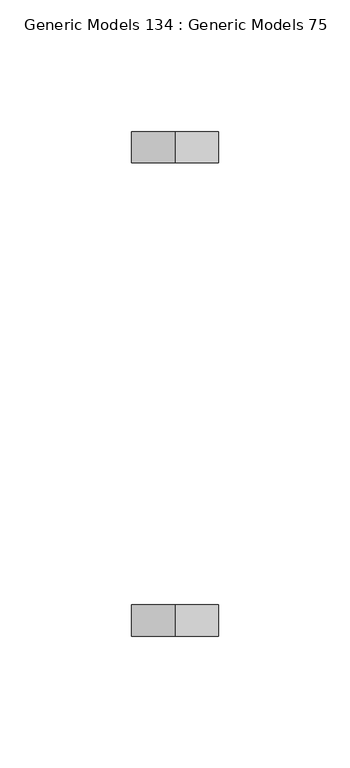
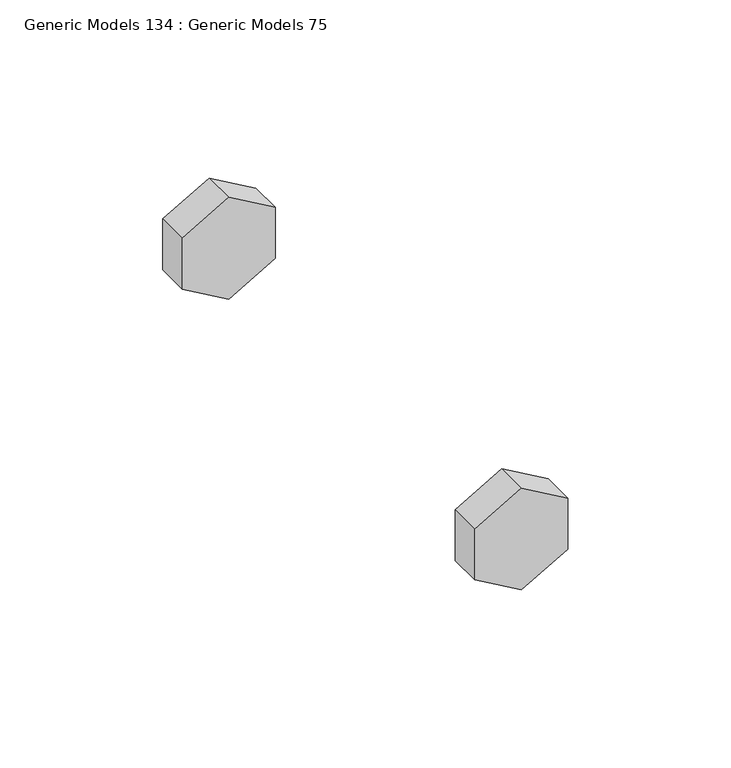
"""IFC4 building model written with IfcOpenShell, lengths in millimetres: proxy geometry, Generic Models 134 : Generic Models 75."""

import ifcopenshell
import ifcopenshell.guid

model = None  # the IFC model being written
_history = None  # IfcOwnerHistory: only IFC2X3 demands one
_inside = {}  # id of a spatial element -> (the spatial element, [elements in it])
_under = {}  # id of a project, library or spatial element -> (it, [spatial elements below it])
_declared = {}  # id of a project -> (the project, [libraries it declares])
_typed = {}  # id of a type object -> (the type object, [elements of that type])
_made_of = {}  # id of a material, layer set ... -> (it, [elements and type objects made of it])


def new_model(schema):
    """Start an empty IFC model of exactly this schema.

    Asked for "IFC4X3", IfcOpenShell would pick the latest addendum, in which some entities
    have other attributes; the version numbers below select the first issue.
    IFC2X3 requires an IfcOwnerHistory on every rooted entity: one is made here for all.
    """
    global model, _history
    if schema == "IFC4X3":
        model = ifcopenshell.file(schema_version=(4, 3, 0, 0))
    else:
        model = ifcopenshell.file(schema=schema)
    _inside.clear()
    _under.clear()
    _declared.clear()
    _typed.clear()
    _made_of.clear()
    _history = None
    if model.schema == "IFC2X3":
        org = make("IfcOrganization", Name="unknown")
        user = make(
            "IfcPersonAndOrganization",
            ThePerson=make("IfcPerson", FamilyName="unknown"),
            TheOrganization=org,
        )
        app = make(
            "IfcApplication",
            ApplicationDeveloper=org,
            Version="unknown",
            ApplicationFullName="unknown",
            ApplicationIdentifier="unknown",
        )
        _history = make(
            "IfcOwnerHistory",
            OwningUser=user,
            OwningApplication=app,
            ChangeAction="ADDED",
            CreationDate=0,
        )
    return model


def make(cls, **values):
    """One entity of the class cls with the attributes given. An attribute that is None is left unset."""
    return model.create_entity(
        cls, **{name: value for name, value in values.items() if value is not None}
    )


def rooted(cls, **values):
    """An entity with a GlobalId (a new one), such as an element, a storey or a relation."""
    return make(cls, GlobalId=ifcopenshell.guid.new(), OwnerHistory=_history, **values)


def si_unit(unit_type, name, prefix=None):
    """IfcSIUnit, for example si_unit("LENGTHUNIT", "METRE", prefix="MILLI")."""
    return make("IfcSIUnit", UnitType=unit_type, Prefix=prefix, Name=name)


def assignment(units):
    """IfcUnitAssignment: the units of a project."""
    return None if units is None else make("IfcUnitAssignment", Units=units)


def point(xyz):
    """IfcCartesianPoint."""
    return None if xyz is None else make("IfcCartesianPoint", Coordinates=xyz)


def direction(xyz):
    """IfcDirection."""
    return None if xyz is None else make("IfcDirection", DirectionRatios=xyz)


def frame(location, z_axis=None, x_axis=None):
    """IfcAxis2Placement3D, a coordinate frame: its origin and axes. An axis left out is left unset."""
    return make(
        "IfcAxis2Placement3D",
        Location=point(location),
        Axis=direction(z_axis),
        RefDirection=direction(x_axis),
    )


def origin():
    """The frame at (0, 0, 0) with its axes left unset."""
    return frame((0.0, 0.0, 0.0))


def place(relative_to, where):
    """IfcLocalPlacement: puts the frame where relative to a parent placement (None: the world)."""
    return make(
        "IfcLocalPlacement", PlacementRelTo=relative_to, RelativePlacement=where
    )


def context(
    kind, dimensions, precision=None, world=None, true_north=None, identifier=None
):
    """IfcGeometricRepresentationContext, for example the 3D "Model" context."""
    return make(
        "IfcGeometricRepresentationContext",
        ContextIdentifier=identifier,
        ContextType=kind,
        CoordinateSpaceDimension=dimensions,
        Precision=precision,
        WorldCoordinateSystem=world,
        TrueNorth=true_north,
    )


def project(units=None, contexts=None):
    """IfcProject with its units and contexts."""
    return rooted(
        "IfcProject",
        Name="project",
        RepresentationContexts=contexts,
        UnitsInContext=assignment(units),
    )


def spatial(cls, under=None, at=None, **own):
    """A site, building, storey or space (cls), placed at a placement, below another one or the project."""
    s = rooted(cls, ObjectPlacement=at, **own)
    if under is not None:
        _under.setdefault(under.id(), (under, []))[1].append(s)
    return s


def polyline(points):
    """IfcPolyline through the points."""
    return make("IfcPolyline", Points=[point(p) for p in points])


def outline(outer, holes=None, kind="AREA"):
    """IfcArbitraryClosedProfileDef: a profile drawn as a closed curve; with holes, ...WithVoids."""
    if holes is None:
        return make("IfcArbitraryClosedProfileDef", ProfileType=kind, OuterCurve=outer)
    return make(
        "IfcArbitraryProfileDefWithVoids",
        ProfileType=kind,
        OuterCurve=outer,
        InnerCurves=holes,
    )


def extrude(swept, where, along, depth):
    """IfcExtrudedAreaSolid: the profile swept, set in the frame where, extruded along a direction by depth."""
    return make(
        "IfcExtrudedAreaSolid",
        SweptArea=swept,
        Position=where,
        ExtrudedDirection=direction(along),
        Depth=depth,
    )


def shape(context_of_items, identifier, shape_type, items):
    """IfcShapeRepresentation: the items that make up one representation, for example the "Body"."""
    return make(
        "IfcShapeRepresentation",
        ContextOfItems=context_of_items,
        RepresentationIdentifier=identifier,
        RepresentationType=shape_type,
        Items=items,
    )


def source(mapping_origin, context_of_items, identifier, shape_type, items):
    """IfcRepresentationMap: a shape defined once, which mapped items show again and again."""
    return make(
        "IfcRepresentationMap",
        MappingOrigin=mapping_origin,
        MappedRepresentation=shape(context_of_items, identifier, shape_type, items),
    )


def transform(
    local_origin,
    x_axis=None,
    y_axis=None,
    z_axis=None,
    scale=None,
    scale2=None,
    scale3=None,
    uniform=True,
):
    """IfcCartesianTransformationOperator3D, or its non-uniform kind. x_axis, y_axis, z_axis: its Axis1, 2, 3."""
    if uniform:
        return make(
            "IfcCartesianTransformationOperator3D",
            Axis1=direction(x_axis),
            Axis2=direction(y_axis),
            LocalOrigin=point(local_origin),
            Scale=scale,
            Axis3=direction(z_axis),
        )
    return make(
        "IfcCartesianTransformationOperator3DnonUniform",
        Axis1=direction(x_axis),
        Axis2=direction(y_axis),
        LocalOrigin=point(local_origin),
        Scale=scale,
        Axis3=direction(z_axis),
        Scale2=scale2,
        Scale3=scale3,
    )


def mapped(mapping_source, mapping_target):
    """IfcMappedItem: shows the shape of a source again, moved by a transform."""
    return make(
        "IfcMappedItem", MappingSource=mapping_source, MappingTarget=mapping_target
    )


def made_of(thing, what):
    """Note that an element or type object is made of a material, layer set ...; save() writes the relation."""
    if what is not None:
        _made_of.setdefault(what.id(), (what, []))[1].append(thing)
    return thing


def element(
    cls,
    number,
    at=None,
    inside=None,
    cuts=None,
    type_object=None,
    material=None,
    context=None,
    identifier="Body",
    shape_type=None,
    held_by="IfcProductDefinitionShape",
    body=None,
    shapes=None,
    **own,
):
    """One element of the class cls, such as IfcWall. Its Tag is "e" and its number.

    at: its placement. inside: the storey or other place that contains it. cuts: it is an
    opening in that element (IfcRelVoidsElement). A single representation is given by context,
    identifier, shape_type and body (its items); several are given by shapes. held_by: the class
    of the entity that holds the representations. save() writes the other relations.
    """
    e = rooted(cls, Tag="e%d" % number, ObjectPlacement=at, **own)
    if body is not None:
        shapes = [shape(context, identifier, shape_type, body)]
    if shapes is not None:
        e.Representation = make(held_by, Representations=shapes)
    if inside is not None:
        _inside.setdefault(inside.id(), (inside, []))[1].append(e)
    if cuts is not None:
        rooted(
            "IfcRelVoidsElement", RelatingBuildingElement=cuts, RelatedOpeningElement=e
        )
    if type_object is not None:
        _typed.setdefault(type_object.id(), (type_object, []))[1].append(e)
    return made_of(e, material)


def aggregate(whole, parts):
    """IfcRelAggregates: a whole, such as a stair, and the parts it consists of."""
    return rooted("IfcRelAggregates", RelatingObject=whole, RelatedObjects=parts)


def save(model, path):
    """Write the relations noted so far, then the file.

    IfcRelAggregates (storeys below a building ...), IfcRelContainedInSpatialStructure (elements
    in a storey), IfcRelDefinesByType, IfcRelAssociatesMaterial and IfcRelDeclares: one each for
    every whole, place, type object, material and project.
    """
    for whole, parts in _under.values():
        aggregate(whole, parts)
    for where, things in _inside.values():
        rooted(
            "IfcRelContainedInSpatialStructure",
            RelatedElements=things,
            RelatingStructure=where,
        )
    for kind, things in _typed.values():
        rooted("IfcRelDefinesByType", RelatedObjects=things, RelatingType=kind)
    for what, things in _made_of.values():
        rooted("IfcRelAssociatesMaterial", RelatedObjects=things, RelatingMaterial=what)
    for by, libraries in _declared.values():
        rooted("IfcRelDeclares", RelatingContext=by, RelatedDefinitions=libraries)
    model.write(path)


def generic_models_134_generic_models_75_c71db7a5(model_context):
    return source(origin(), model_context, "Body", "SweptSolid", [
        extrude(outline(polyline([(269389.225, 31991.9073871), (269408.275, 31991.9073871), (269417.8, 31975.4096032), (269408.275, 31958.9118192), (269389.225, 31958.9118192), (269379.7, 31975.4096032), (269389.225, 31991.9073871)])), frame((0.0, 33979.5460924, 0.0), z_axis=(0.0, 1.0, 0.0), x_axis=(0.0, 0.0, 1.0)), (0.0, 0.0, 1.0), 11.90625),
        extrude(outline(polyline([(269389.225, 31991.9073871), (269408.275, 31991.9073871), (269417.8, 31975.4096032), (269408.275, 31958.9118192), (269389.225, 31958.9118192), (269379.7, 31975.4096032), (269389.225, 31991.9073871)])), frame((0.0, 34159.3304674, 0.0), z_axis=(0.0, 1.0, 0.0), x_axis=(0.0, 0.0, 1.0)), (0.0, 0.0, 1.0), 11.90625),
    ])


if __name__ == "__main__":
    model = new_model("IFC4")
    model_context = context("Model", 3, world=origin())
    ifc_project = project(units=[si_unit("LENGTHUNIT", "METRE", prefix="MILLI")], contexts=[model_context])
    site = spatial("IfcSite", under=ifc_project)
    building = spatial("IfcBuilding", under=site)
    placement = place(None, origin())
    generic_models_134_generic_models_75_shape = generic_models_134_generic_models_75_c71db7a5(model_context)
    element("IfcBuildingElementProxy", 1, Name="Generic Models 134 : Generic Models 75", ObjectType="Generic Models 134 : Generic Models 75", at=placement, inside=building, context=model_context, shape_type="MappedRepresentation", body=[
        mapped(generic_models_134_generic_models_75_shape, transform((0.0, 0.0, 0.0), x_axis=(1.0, 0.0, 0.0), y_axis=(0.0, 1.0, 0.0), z_axis=(0.0, 0.0, 1.0))),
    ])
    save(model, "model.ifc")
